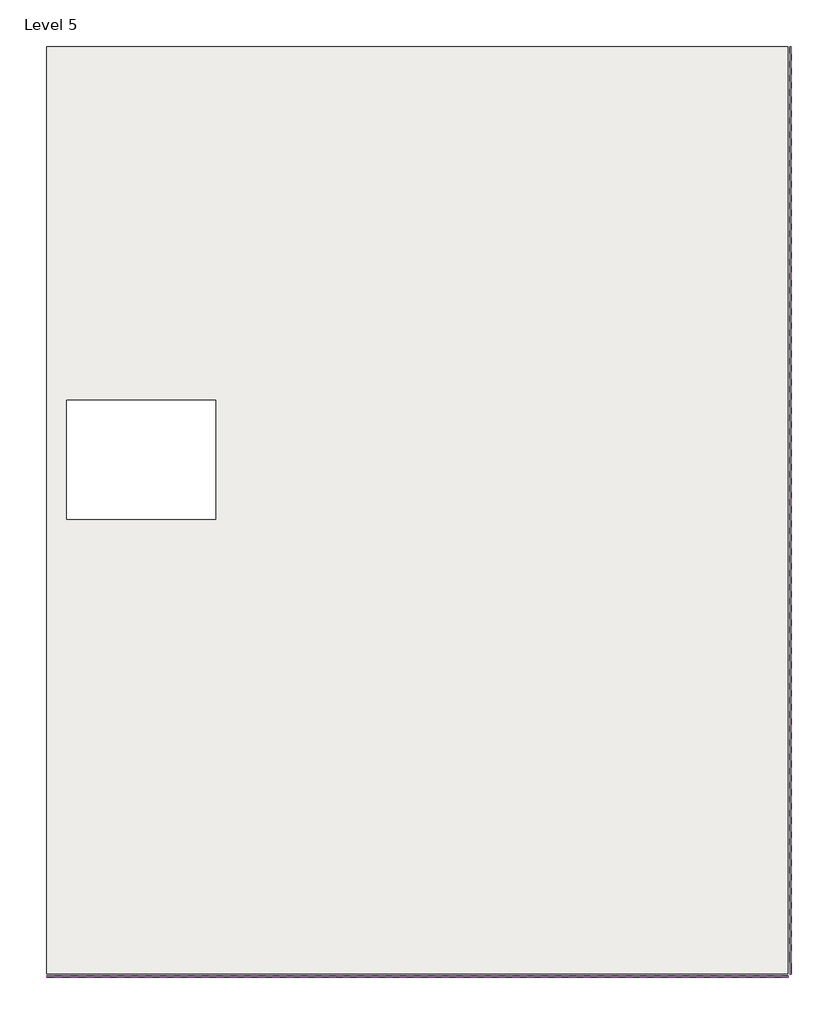
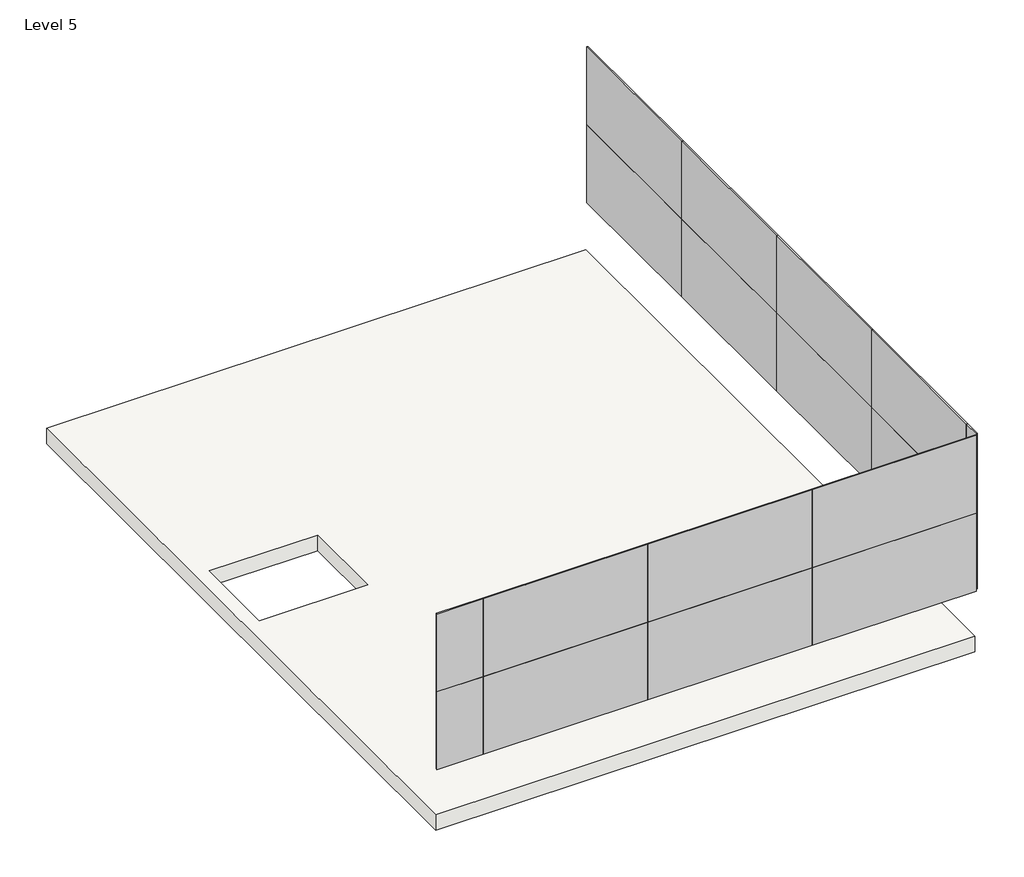
# One storey: 18 plates, 1 slab.
"""IFC4 building model written with IfcOpenShell, lengths in millimetres."""

import ifcopenshell
import ifcopenshell.guid

model = None  # the IFC model being written
_history = None  # IfcOwnerHistory: only IFC2X3 demands one
_inside = {}  # id of a spatial element -> (the spatial element, [elements in it])
_under = {}  # id of a project, library or spatial element -> (it, [spatial elements below it])
_declared = {}  # id of a project -> (the project, [libraries it declares])
_typed = {}  # id of a type object -> (the type object, [elements of that type])
_made_of = {}  # id of a material, layer set ... -> (it, [elements and type objects made of it])


def new_model(schema):
    """Start an empty IFC model of exactly this schema.

    Asked for "IFC4X3", IfcOpenShell would pick the latest addendum, in which some entities
    have other attributes; the version numbers below select the first issue.
    IFC2X3 requires an IfcOwnerHistory on every rooted entity: one is made here for all.
    """
    global model, _history
    if schema == "IFC4X3":
        model = ifcopenshell.file(schema_version=(4, 3, 0, 0))
    else:
        model = ifcopenshell.file(schema=schema)
    _inside.clear()
    _under.clear()
    _declared.clear()
    _typed.clear()
    _made_of.clear()
    _history = None
    if model.schema == "IFC2X3":
        org = make("IfcOrganization", Name="unknown")
        user = make(
            "IfcPersonAndOrganization",
            ThePerson=make("IfcPerson", FamilyName="unknown"),
            TheOrganization=org,
        )
        app = make(
            "IfcApplication",
            ApplicationDeveloper=org,
            Version="unknown",
            ApplicationFullName="unknown",
            ApplicationIdentifier="unknown",
        )
        _history = make(
            "IfcOwnerHistory",
            OwningUser=user,
            OwningApplication=app,
            ChangeAction="ADDED",
            CreationDate=0,
        )
    return model


def make(cls, **values):
    """One entity of the class cls with the attributes given. An attribute that is None is left unset."""
    return model.create_entity(
        cls, **{name: value for name, value in values.items() if value is not None}
    )


def rooted(cls, **values):
    """An entity with a GlobalId (a new one), such as an element, a storey or a relation."""
    return make(cls, GlobalId=ifcopenshell.guid.new(), OwnerHistory=_history, **values)


def si_unit(unit_type, name, prefix=None):
    """IfcSIUnit, for example si_unit("LENGTHUNIT", "METRE", prefix="MILLI")."""
    return make("IfcSIUnit", UnitType=unit_type, Prefix=prefix, Name=name)


def assignment(units):
    """IfcUnitAssignment: the units of a project."""
    return None if units is None else make("IfcUnitAssignment", Units=units)


def point(xyz):
    """IfcCartesianPoint."""
    return None if xyz is None else make("IfcCartesianPoint", Coordinates=xyz)


def direction(xyz):
    """IfcDirection."""
    return None if xyz is None else make("IfcDirection", DirectionRatios=xyz)


def frame(location, z_axis=None, x_axis=None):
    """IfcAxis2Placement3D, a coordinate frame: its origin and axes. An axis left out is left unset."""
    return make(
        "IfcAxis2Placement3D",
        Location=point(location),
        Axis=direction(z_axis),
        RefDirection=direction(x_axis),
    )


def origin():
    """The frame at (0, 0, 0) with its axes left unset."""
    return frame((0.0, 0.0, 0.0))


def origin_with_axes():
    """The frame at (0, 0, 0) with the z axis (0, 0, 1) and the x axis (1, 0, 0) written out."""
    return frame((0.0, 0.0, 0.0), z_axis=(0.0, 0.0, 1.0), x_axis=(1.0, 0.0, 0.0))


def place(relative_to, where):
    """IfcLocalPlacement: puts the frame where relative to a parent placement (None: the world)."""
    return make(
        "IfcLocalPlacement", PlacementRelTo=relative_to, RelativePlacement=where
    )


def context(
    kind, dimensions, precision=None, world=None, true_north=None, identifier=None
):
    """IfcGeometricRepresentationContext, for example the 3D "Model" context."""
    return make(
        "IfcGeometricRepresentationContext",
        ContextIdentifier=identifier,
        ContextType=kind,
        CoordinateSpaceDimension=dimensions,
        Precision=precision,
        WorldCoordinateSystem=world,
        TrueNorth=true_north,
    )


def project(units=None, contexts=None):
    """IfcProject with its units and contexts."""
    return rooted(
        "IfcProject",
        Name="project",
        RepresentationContexts=contexts,
        UnitsInContext=assignment(units),
    )


def spatial(cls, under=None, at=None, **own):
    """A site, building, storey or space (cls), placed at a placement, below another one or the project."""
    s = rooted(cls, ObjectPlacement=at, **own)
    if under is not None:
        _under.setdefault(under.id(), (under, []))[1].append(s)
    return s


def polyline(points):
    """IfcPolyline through the points."""
    return make("IfcPolyline", Points=[point(p) for p in points])


def outline(outer, holes=None, kind="AREA"):
    """IfcArbitraryClosedProfileDef: a profile drawn as a closed curve; with holes, ...WithVoids."""
    if holes is None:
        return make("IfcArbitraryClosedProfileDef", ProfileType=kind, OuterCurve=outer)
    return make(
        "IfcArbitraryProfileDefWithVoids",
        ProfileType=kind,
        OuterCurve=outer,
        InnerCurves=holes,
    )


def extrude(swept, where, along, depth):
    """IfcExtrudedAreaSolid: the profile swept, set in the frame where, extruded along a direction by depth."""
    return make(
        "IfcExtrudedAreaSolid",
        SweptArea=swept,
        Position=where,
        ExtrudedDirection=direction(along),
        Depth=depth,
    )


def shape(context_of_items, identifier, shape_type, items):
    """IfcShapeRepresentation: the items that make up one representation, for example the "Body"."""
    return make(
        "IfcShapeRepresentation",
        ContextOfItems=context_of_items,
        RepresentationIdentifier=identifier,
        RepresentationType=shape_type,
        Items=items,
    )


def source(mapping_origin, context_of_items, identifier, shape_type, items):
    """IfcRepresentationMap: a shape defined once, which mapped items show again and again."""
    return make(
        "IfcRepresentationMap",
        MappingOrigin=mapping_origin,
        MappedRepresentation=shape(context_of_items, identifier, shape_type, items),
    )


def transform(
    local_origin,
    x_axis=None,
    y_axis=None,
    z_axis=None,
    scale=None,
    scale2=None,
    scale3=None,
    uniform=True,
):
    """IfcCartesianTransformationOperator3D, or its non-uniform kind. x_axis, y_axis, z_axis: its Axis1, 2, 3."""
    if uniform:
        return make(
            "IfcCartesianTransformationOperator3D",
            Axis1=direction(x_axis),
            Axis2=direction(y_axis),
            LocalOrigin=point(local_origin),
            Scale=scale,
            Axis3=direction(z_axis),
        )
    return make(
        "IfcCartesianTransformationOperator3DnonUniform",
        Axis1=direction(x_axis),
        Axis2=direction(y_axis),
        LocalOrigin=point(local_origin),
        Scale=scale,
        Axis3=direction(z_axis),
        Scale2=scale2,
        Scale3=scale3,
    )


def mapped(mapping_source, mapping_target):
    """IfcMappedItem: shows the shape of a source again, moved by a transform."""
    return make(
        "IfcMappedItem", MappingSource=mapping_source, MappingTarget=mapping_target
    )


def made_of(thing, what):
    """Note that an element or type object is made of a material, layer set ...; save() writes the relation."""
    if what is not None:
        _made_of.setdefault(what.id(), (what, []))[1].append(thing)
    return thing


def element(
    cls,
    number,
    at=None,
    inside=None,
    cuts=None,
    type_object=None,
    material=None,
    context=None,
    identifier="Body",
    shape_type=None,
    held_by="IfcProductDefinitionShape",
    body=None,
    shapes=None,
    **own,
):
    """One element of the class cls, such as IfcWall. Its Tag is "e" and its number.

    at: its placement. inside: the storey or other place that contains it. cuts: it is an
    opening in that element (IfcRelVoidsElement). A single representation is given by context,
    identifier, shape_type and body (its items); several are given by shapes. held_by: the class
    of the entity that holds the representations. save() writes the other relations.
    """
    e = rooted(cls, Tag="e%d" % number, ObjectPlacement=at, **own)
    if body is not None:
        shapes = [shape(context, identifier, shape_type, body)]
    if shapes is not None:
        e.Representation = make(held_by, Representations=shapes)
    if inside is not None:
        _inside.setdefault(inside.id(), (inside, []))[1].append(e)
    if cuts is not None:
        rooted(
            "IfcRelVoidsElement", RelatingBuildingElement=cuts, RelatedOpeningElement=e
        )
    if type_object is not None:
        _typed.setdefault(type_object.id(), (type_object, []))[1].append(e)
    return made_of(e, material)


def aggregate(whole, parts):
    """IfcRelAggregates: a whole, such as a stair, and the parts it consists of."""
    return rooted("IfcRelAggregates", RelatingObject=whole, RelatedObjects=parts)


def save(model, path):
    """Write the relations noted so far, then the file.

    IfcRelAggregates (storeys below a building ...), IfcRelContainedInSpatialStructure (elements
    in a storey), IfcRelDefinesByType, IfcRelAssociatesMaterial and IfcRelDeclares: one each for
    every whole, place, type object, material and project.
    """
    for whole, parts in _under.values():
        aggregate(whole, parts)
    for where, things in _inside.values():
        rooted(
            "IfcRelContainedInSpatialStructure",
            RelatedElements=things,
            RelatingStructure=where,
        )
    for kind, things in _typed.values():
        rooted("IfcRelDefinesByType", RelatedObjects=things, RelatingType=kind)
    for what, things in _made_of.values():
        rooted("IfcRelAssociatesMaterial", RelatedObjects=things, RelatingMaterial=what)
    for by, libraries in _declared.values():
        rooted("IfcRelDeclares", RelatingContext=by, RelatedDefinitions=libraries)
    model.write(path)


def system_panel_glazed_1e57f9bb(model_context):
    return source(origin(), model_context, "Body", "SweptSolid", [
        extrude(outline(polyline([(1524.0000002, 19.05), (-1524.0000002, 19.05), (-1524.0000002, 44.45), (1524.0000002, 44.45), (1524.0000002, 19.05)])), origin_with_axes(), (0.0, 0.0, 1.0), 1524.0),
    ])


def system_panel_glazed_ccfd9adb(model_context):
    return source(origin(), model_context, "Body", "SweptSolid", [
        extrude(outline(polyline([(427.9999998, 19.05), (-427.9999998, 19.05), (-427.9999998, 44.45), (427.9999998, 44.45), (427.9999998, 19.05)])), origin_with_axes(), (0.0, 0.0, 1.0), 1524.0),
    ])


def system_panel_glazed_88f24eba(model_context):
    return source(origin(), model_context, "Body", "SweptSolid", [
        extrude(outline(polyline([(153.9999998, 19.05), (-153.9999998, 19.05), (-153.9999998, 44.45), (153.9999998, 44.45), (153.9999998, 19.05)])), origin_with_axes(), (0.0, 0.0, 1.0), 1524.0),
    ])


model = new_model("IFC4")

# Units and contexts
model_context = context("Model", 3, world=origin())
ifc_project = project(units=[si_unit("LENGTHUNIT", "METRE", prefix="MILLI")], contexts=[model_context])

# Site, building, storey
site = spatial("IfcSite", under=ifc_project)
building = spatial("IfcBuilding", under=site)
storey = spatial("IfcBuildingStorey", under=building, Name="Level 5", Elevation=12800.0)

# Plates
placement = place(None, origin())
system_panel_glazed_shape = system_panel_glazed_1e57f9bb(model_context)
element("IfcPlate", 1, ObjectType="System Panel : Glazed", at=placement, inside=storey, context=model_context, shape_type="MappedRepresentation", body=[
    mapped(system_panel_glazed_shape, transform((2137.6340362, 1399.6955828, 13716.0), x_axis=(-1.0, 0.0, 0.0), y_axis=(0.0, -1.0, 0.0), z_axis=(0.0, 0.0, 1.0))),
])
element("IfcPlate", 2, ObjectType="System Panel : Glazed", at=placement, inside=storey, context=model_context, shape_type="MappedRepresentation", body=[
    mapped(system_panel_glazed_shape, transform((-910.3659639, 1399.6955828, 13716.0), x_axis=(-1.0, 0.0, 0.0), y_axis=(0.0, -1.0, 0.0), z_axis=(0.0, 0.0, 1.0))),
])
element("IfcPlate", 3, ObjectType="System Panel : Glazed", at=placement, inside=storey, context=model_context, shape_type="MappedRepresentation", body=[
    mapped(system_panel_glazed_shape, transform((-3958.3659639, 1399.6955828, 13716.0), x_axis=(-1.0, 0.0, 0.0), y_axis=(0.0, -1.0, 0.0), z_axis=(0.0, 0.0, 1.0))),
])
element("IfcPlate", 4, ObjectType="System Panel : Glazed", at=placement, inside=storey, context=model_context, shape_type="MappedRepresentation", body=[
    mapped(system_panel_glazed_shape, transform((2137.6340362, 1399.6955828, 15240.0), x_axis=(-1.0, 0.0, 0.0), y_axis=(0.0, -1.0, 0.0), z_axis=(0.0, 0.0, 1.0))),
])
element("IfcPlate", 5, ObjectType="System Panel : Glazed", at=placement, inside=storey, context=model_context, shape_type="MappedRepresentation", body=[
    mapped(system_panel_glazed_shape, transform((-910.3659639, 1399.6955828, 15240.0), x_axis=(-1.0, 0.0, 0.0), y_axis=(0.0, -1.0, 0.0), z_axis=(0.0, 0.0, 1.0))),
])
element("IfcPlate", 6, ObjectType="System Panel : Glazed", at=placement, inside=storey, context=model_context, shape_type="MappedRepresentation", body=[
    mapped(system_panel_glazed_shape, transform((-3958.3659639, 1399.6955828, 15240.0), x_axis=(-1.0, 0.0, 0.0), y_axis=(0.0, -1.0, 0.0), z_axis=(0.0, 0.0, 1.0))),
])
element("IfcPlate", 7, ObjectType="System Panel : Glazed", at=placement, inside=storey, context=model_context, shape_type="MappedRepresentation", body=[
    mapped(system_panel_glazed_shape, transform((3661.6340364, 12375.6955827, 13716.0), x_axis=(0.0, -1.0, 0.0), y_axis=(1.0, 0.0, 0.0), z_axis=(0.0, 0.0, 1.0))),
])
element("IfcPlate", 8, ObjectType="System Panel : Glazed", at=placement, inside=storey, context=model_context, shape_type="MappedRepresentation", body=[
    mapped(system_panel_glazed_shape, transform((3661.6340364, 9327.6955825, 13716.0), x_axis=(0.0, -1.0, 0.0), y_axis=(1.0, 0.0, 0.0), z_axis=(0.0, 0.0, 1.0))),
])
element("IfcPlate", 9, ObjectType="System Panel : Glazed", at=placement, inside=storey, context=model_context, shape_type="MappedRepresentation", body=[
    mapped(system_panel_glazed_shape, transform((3661.6340364, 6279.6955825, 13716.0), x_axis=(0.0, -1.0, 0.0), y_axis=(1.0, 0.0, 0.0), z_axis=(0.0, 0.0, 1.0))),
])
element("IfcPlate", 10, ObjectType="System Panel : Glazed", at=placement, inside=storey, context=model_context, shape_type="MappedRepresentation", body=[
    mapped(system_panel_glazed_shape, transform((3661.6340364, 3231.6955825, 13716.0), x_axis=(0.0, -1.0, 0.0), y_axis=(1.0, 0.0, 0.0), z_axis=(0.0, 0.0, 1.0))),
])
element("IfcPlate", 11, ObjectType="System Panel : Glazed", at=placement, inside=storey, context=model_context, shape_type="MappedRepresentation", body=[
    mapped(system_panel_glazed_shape, transform((3661.6340364, 12375.6955827, 15240.0), x_axis=(0.0, -1.0, 0.0), y_axis=(1.0, 0.0, 0.0), z_axis=(0.0, 0.0, 1.0))),
])
element("IfcPlate", 12, ObjectType="System Panel : Glazed", at=placement, inside=storey, context=model_context, shape_type="MappedRepresentation", body=[
    mapped(system_panel_glazed_shape, transform((3661.6340364, 9327.6955825, 15240.0), x_axis=(0.0, -1.0, 0.0), y_axis=(1.0, 0.0, 0.0), z_axis=(0.0, 0.0, 1.0))),
])
element("IfcPlate", 13, ObjectType="System Panel : Glazed", at=placement, inside=storey, context=model_context, shape_type="MappedRepresentation", body=[
    mapped(system_panel_glazed_shape, transform((3661.6340364, 6279.6955825, 15240.0), x_axis=(0.0, -1.0, 0.0), y_axis=(1.0, 0.0, 0.0), z_axis=(0.0, 0.0, 1.0))),
])
element("IfcPlate", 14, ObjectType="System Panel : Glazed", at=placement, inside=storey, context=model_context, shape_type="MappedRepresentation", body=[
    mapped(system_panel_glazed_shape, transform((3661.6340364, 3231.6955825, 15240.0), x_axis=(0.0, -1.0, 0.0), y_axis=(1.0, 0.0, 0.0), z_axis=(0.0, 0.0, 1.0))),
])
system_panel_glazed_2_shape = system_panel_glazed_ccfd9adb(model_context)
element("IfcPlate", 15, ObjectType="System Panel : Glazed", at=placement, inside=storey, context=model_context, shape_type="MappedRepresentation", body=[
    mapped(system_panel_glazed_2_shape, transform((-5910.3659638, 1399.6955828, 13716.0), x_axis=(-1.0, 0.0, 0.0), y_axis=(0.0, -1.0, 0.0), z_axis=(0.0, 0.0, 1.0))),
])
element("IfcPlate", 16, ObjectType="System Panel : Glazed", at=placement, inside=storey, context=model_context, shape_type="MappedRepresentation", body=[
    mapped(system_panel_glazed_2_shape, transform((-5910.3659638, 1399.6955828, 15240.0), x_axis=(-1.0, 0.0, 0.0), y_axis=(0.0, -1.0, 0.0), z_axis=(0.0, 0.0, 1.0))),
])
system_panel_glazed_3_shape = system_panel_glazed_88f24eba(model_context)
element("IfcPlate", 17, ObjectType="System Panel : Glazed", at=placement, inside=storey, context=model_context, shape_type="MappedRepresentation", body=[
    mapped(system_panel_glazed_3_shape, transform((3661.6340364, 1553.6955827, 13716.0), x_axis=(0.0, -1.0, 0.0), y_axis=(1.0, 0.0, 0.0), z_axis=(0.0, 0.0, 1.0))),
])
element("IfcPlate", 18, ObjectType="System Panel : Glazed", at=placement, inside=storey, context=model_context, shape_type="MappedRepresentation", body=[
    mapped(system_panel_glazed_3_shape, transform((3661.6340364, 1553.6955827, 15240.0), x_axis=(0.0, -1.0, 0.0), y_axis=(1.0, 0.0, 0.0), z_axis=(0.0, 0.0, 1.0))),
])

# Slab
element("IfcSlab", 19, ObjectType="Generic - 12\"", at=placement, inside=storey, context=model_context, shape_type="SweptSolid", body=[
    extrude(outline(polyline([(-6335.3659636, 1402.6955828), (-6335.3659636, 13896.6955828), (3658.6340364, 13896.6955828), (3658.6340364, 1402.6955828), (-6335.3659636, 1402.6955828)]), holes=[polyline([(-4059.8993101, 7527.9023719), (-4059.8993101, 9133.9023719), (-6065.8993101, 9133.9023719), (-6065.8993101, 7527.9023719), (-4059.8993101, 7527.9023719)])]), frame((0.0, 0.0, 12495.2), z_axis=(0.0, 0.0, 1.0), x_axis=(1.0, 0.0, 0.0)), (0.0, 0.0, 1.0), 304.8),
])

save(model, "model.ifc")

# Revit data of these elements
# Type "System Panel : Glazed"
#   Construction Type Id = "GSP4R"
#   Analytic Construction = "1/8 in Pilkington single glazing"
#   Visual Light Transmittance = 0.9
#   Solar Heat Gain Coefficient = 0.86
#   Heat Transfer Coefficient (U) = 6.7069 W/(m²·K)
# Type "Generic - 12\""
#   Assembly Code = "B1010"
#   Function = 0
#   Layers, outside or top first: 0.3048 m no material (function 1)
# Elements 1, 2, 3, 4, 5, 6, 7, 8, 9, 10, 11, 12, 13, 14, 15, 16, 17, 18 (IfcPlate, "System Panel : Glazed")
#   Phase Created = New Construction
#   Materials on its faces: "Glass"
# Element 19 (IfcSlab, "Generic - 12\"")
#   built-in parameter 1001955 = -1.5708 (stored number, unit not read)
#   Height Offset From Level = 0.00 m
#   Phase Created = New Construction
#   Materials on its faces: "Default Floor"
# Materials
#   "Glass": class "Glass", colour RGB 0 128 192, transparency 0.75, Description = "Soda Lime Glass", Cost = 0
#   "Default Floor": class "Miscellaneous", colour RGB 128 128 128, transparency 0, Cost = 0
